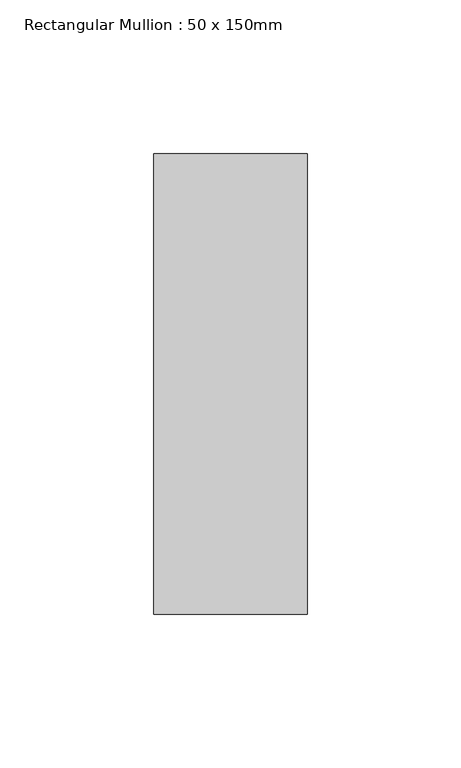
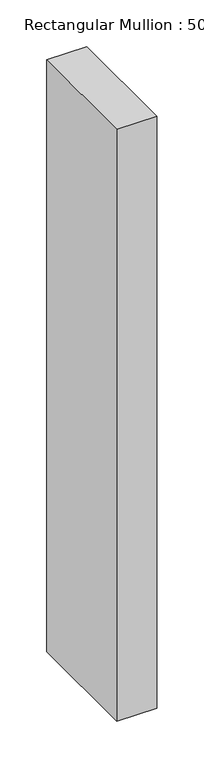
"""IFC4 building model written with IfcOpenShell, lengths in millimetres: member geometry, Rectangular Mullion : 50 x 150mm."""

from ifc_helpers import new_model, si_unit, frame, origin, place, context, project, spatial, polyline, outline, extrude, source, transform, mapped, element, save


def rectangular_mullion_50_x_150mm_5dc04e1f(model_context):
    return source(origin(), model_context, "Body", "SweptSolid", [
        extrude(outline(polyline([(0.0, 75.0), (0.0, -75.0), (-50.0, -75.0), (-50.0, 75.0), (0.0, 75.0)])), frame((0.0, 0.0, -775.0), z_axis=(0.0, 0.0, 1.0), x_axis=(1.0, 0.0, 0.0)), (0.0, 0.0, 1.0), 775.0),
    ])


if __name__ == "__main__":
    model = new_model("IFC4")
    model_context = context("Model", 3, world=origin())
    ifc_project = project(units=[si_unit("LENGTHUNIT", "METRE", prefix="MILLI")], contexts=[model_context])
    site = spatial("IfcSite", under=ifc_project)
    building = spatial("IfcBuilding", under=site)
    placement = place(None, origin())
    rectangular_mullion_50_x_150mm_shape = rectangular_mullion_50_x_150mm_5dc04e1f(model_context)
    element("IfcMember", 1, ObjectType="Rectangular Mullion : 50 x 150mm", at=placement, inside=building, context=model_context, shape_type="MappedRepresentation", body=[
        mapped(rectangular_mullion_50_x_150mm_shape, transform((0.0, 0.0, 0.0), x_axis=(1.0, 0.0, 0.0), y_axis=(0.0, 1.0, 0.0), z_axis=(0.0, 0.0, 1.0))),
    ])
    save(model, "model.ifc")

# Revit data of these elements
# Type "Rectangular Mullion : 50 x 150mm"
#   built-in parameter 1007304 = 0.492126 (stored number, unit not read)
#   built-in parameter 1007301 = 0.082021 (stored number, unit not read)
#   built-in parameter 1007300 = 0.082021 (stored number, unit not read)
# Element 1 (IfcMember, "Rectangular Mullion : 50 x 150mm")
#   Materials on its faces: "Metal - Aluminium"
# Materials
#   "Metal - Aluminium": class "Metal", colour RGB 247 247 247, transparency 0
